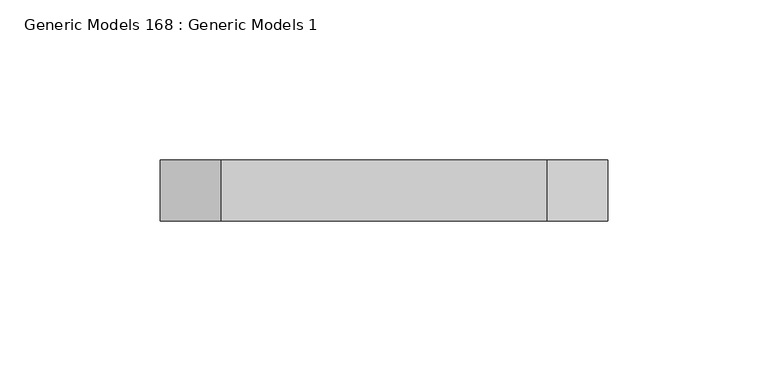
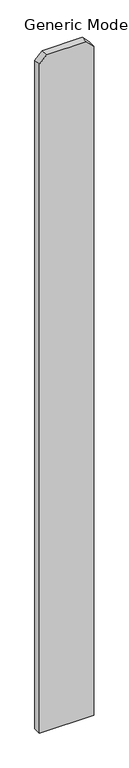
"""IFC4 building model written with IfcOpenShell, lengths in millimetres: proxy geometry, Generic Models 168 : Generic Models 1."""

from ifc_helpers import new_model, si_unit, frame, origin, place, context, project, spatial, polyline, outline, extrude, source, transform, mapped, element, save


def generic_models_168_generic_models_1_c8465e2c(model_context):
    return source(origin(), model_context, "Body", "SweptSolid", [
        extrude(outline(polyline([(76.2, -249200.9875), (1885.95, -249200.9875), (1905.0, -249220.0375), (1905.0, -249321.6375), (1885.95, -249340.6875), (76.2, -249340.6875), (76.2, -249200.9875)])), frame((0.0, 547.6875, 0.0), z_axis=(0.0, 1.0, 0.0), x_axis=(0.0, 0.0, 1.0)), (0.0, 0.0, 1.0), 19.05),
    ])


if __name__ == "__main__":
    model = new_model("IFC4")
    model_context = context("Model", 3, world=origin())
    ifc_project = project(units=[si_unit("LENGTHUNIT", "METRE", prefix="MILLI")], contexts=[model_context])
    site = spatial("IfcSite", under=ifc_project)
    building = spatial("IfcBuilding", under=site)
    placement = place(None, origin())
    generic_models_168_generic_models_1_shape = generic_models_168_generic_models_1_c8465e2c(model_context)
    element("IfcBuildingElementProxy", 1, Name="Generic Models 168 : Generic Models 1", ObjectType="Generic Models 168 : Generic Models 1", at=placement, inside=building, context=model_context, shape_type="MappedRepresentation", body=[
        mapped(generic_models_168_generic_models_1_shape, transform((0.0, 0.0, 0.0), x_axis=(1.0, 0.0, 0.0), y_axis=(0.0, 1.0, 0.0), z_axis=(0.0, 0.0, 1.0))),
    ])
    save(model, "model.ifc")

# Revit data of these elements
# Element 1 (IfcBuildingElementProxy, "Generic Models 168 : Generic Models 1")
#   Materials on its faces: "VERTICAL 1X6 CEDAR PLANKS W/ CLEAR WOOD SEALER"
# Materials
#   "VERTICAL 1X6 CEDAR PLANKS W/ CLEAR WOOD SEALER": class "Wood", colour RGB 234 198 147, transparency 0, Description = "Pinus Echinata", Cost = 0
